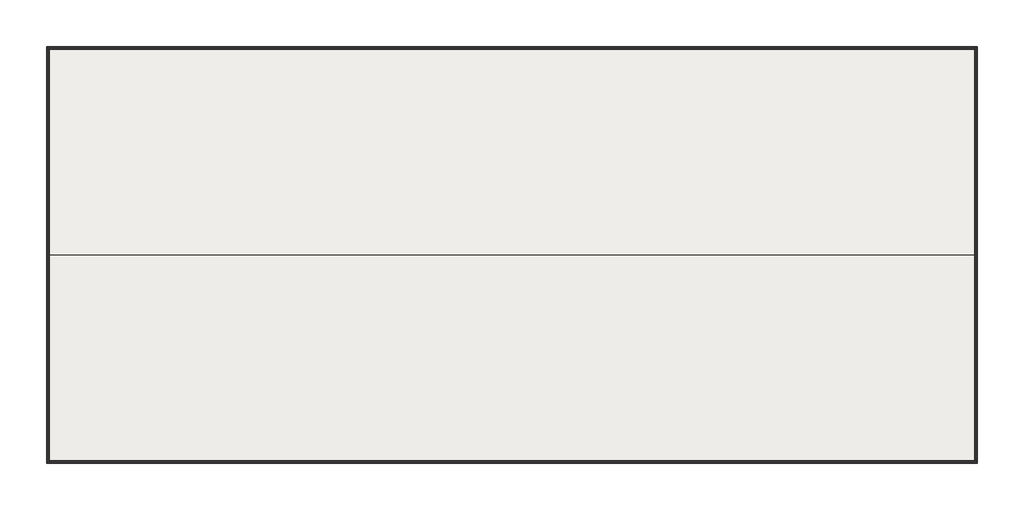
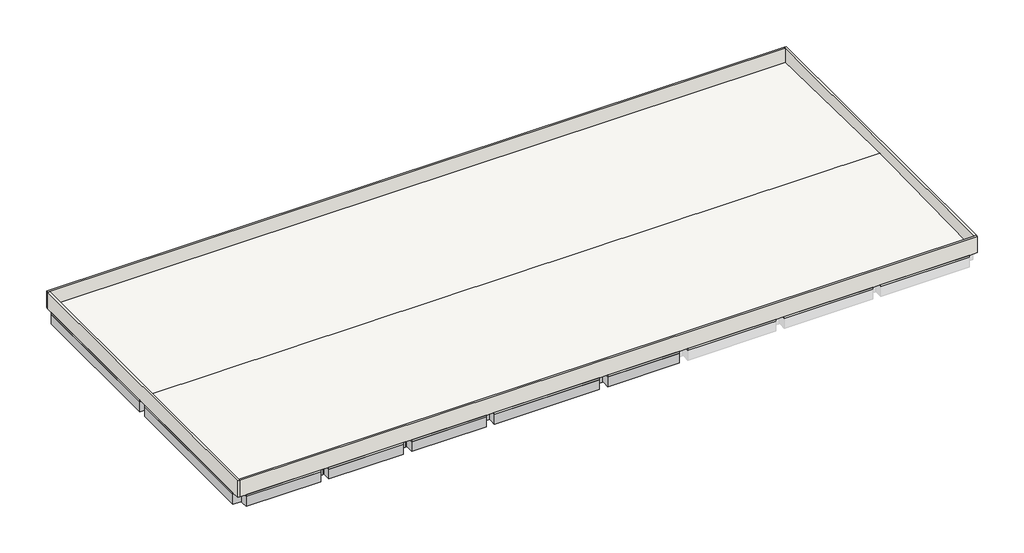
# One storey, part 1 of 2: 21 beams, 4 walls, 1 roof, 1 slab.
"""IFC4 building model written with IfcOpenShell, lengths in millimetres."""

from ifc_helpers import new_model, si_unit, frame, origin, place, context, project, spatial, polyline, outline, extrude, faceted_brep, element, save

model = new_model("IFC4")

# Units and contexts
model_context = context("Model", 3, world=origin())
ifc_project = project(units=[si_unit("LENGTHUNIT", "METRE", prefix="MILLI")], contexts=[model_context])

# Site, building, storey
site = spatial("IfcSite", under=ifc_project)
building = spatial("IfcBuilding", under=site)
storey = spatial("IfcBuildingStorey", under=building, Name="TOC", Elevation=7649.9618634)

# Beams
placement = place(None, origin())
element("IfcBeam", 1, ObjectType="RC Beam_Rectangular : H_SB_AR_S16_B600xH900_RG4", at=placement, inside=storey, context=model_context, shape_type="Brep", body=[
    faceted_brep([(300.0, 12499.5208589, 6749.9618634), (300.0, 12099.5208589, 6749.9618634), (300.0, 11899.5208589, 6749.9618634), (300.0, 11899.5208589, 7499.9618634), (300.0, 12499.5208589, 7499.9618634), (5700.0, 11899.5208589, 6749.9618634), (5700.0, 12099.5208589, 6749.9618634), (5700.0, 12499.5208589, 6749.9618634), (5700.0, 12499.5208589, 7499.9618634), (5700.0, 11899.5208589, 7499.9618634), (426.0, 11899.5208589, 7499.9618634), (2800.0, 11899.5208589, 7499.9618634), (3200.0, 11899.5208589, 7499.9618634), (3200.0, 12499.5208589, 7499.9618634), (2800.0, 12499.5208589, 7499.9618634), (426.0, 12499.5208589, 7499.9618634), (2800.0, 11899.5208589, 6749.9618634), (3200.0, 11899.5208589, 6749.9618634), (426.0, 12499.5208589, 6749.9618634), (2800.0, 12499.5208589, 6749.9618634), (3200.0, 12499.5208589, 6749.9618634)], [[[0, 1, 2, 3, 4]], [[5, 6, 7, 8, 9]], [[4, 3, 10, 11, 12, 9, 8, 13, 14, 15]], [[2, 16, 17, 5, 9, 12, 11, 10, 3]], [[2, 1, 0, 18, 19, 20, 7, 6, 5, 17, 16]], [[7, 20, 19, 18, 0, 4, 15, 14, 13, 8]]]),
])
element("IfcBeam", 2, ObjectType="RC Beam_Rectangular : H_SB_AR_S16_B600xH900_RG4", at=placement, inside=storey, context=model_context, shape_type="Brep", body=[
    faceted_brep([(6300.0, 12499.5208589, 6749.9618634), (6300.0, 12099.5208589, 6749.9618634), (6300.0, 11899.5208589, 6749.9618634), (6300.0, 11899.5208589, 7499.9618634), (6300.0, 12499.5208589, 7499.9618634), (11700.0, 11899.5208589, 6749.9618634), (11700.0, 12099.5208589, 6749.9618634), (11700.0, 12499.5208589, 6749.9618634), (11700.0, 12499.5208589, 7499.9618634), (11700.0, 11899.5208589, 7499.9618634), (8800.0, 11899.5208589, 7499.9618634), (9200.0, 11899.5208589, 7499.9618634), (9200.0, 12499.5208589, 7499.9618634), (8800.0, 12499.5208589, 7499.9618634), (8800.0, 11899.5208589, 6749.9618634), (9200.0, 11899.5208589, 6749.9618634), (8800.0, 12499.5208589, 6749.9618634), (9200.0, 12499.5208589, 6749.9618634)], [[[0, 1, 2, 3, 4]], [[5, 6, 7, 8, 9]], [[4, 3, 10, 11, 9, 8, 12, 13]], [[2, 14, 15, 5, 9, 11, 10, 3]], [[2, 1, 0, 16, 17, 7, 6, 5, 15, 14]], [[7, 17, 16, 0, 4, 13, 12, 8]]]),
])
element("IfcBeam", 3, ObjectType="RC Beam_Rectangular : H_SB_AR_S16_B600xH900_RG4", at=placement, inside=storey, context=model_context, shape_type="Brep", body=[
    faceted_brep([(12300.0, 12499.5208589, 6749.9618634), (12300.0, 12099.5208589, 6749.9618634), (12300.0, 11899.5208589, 6749.9618634), (12300.0, 11899.5208589, 7499.9618634), (12300.0, 12499.5208589, 7499.9618634), (17700.0, 11899.5208589, 6749.9618634), (17700.0, 12099.5208589, 6749.9618634), (17700.0, 12499.5208589, 6749.9618634), (17700.0, 12499.5208589, 7499.9618634), (17700.0, 11899.5208589, 7499.9618634), (14800.0, 11899.5208589, 7499.9618634), (15200.0, 11899.5208589, 7499.9618634), (15200.0, 12499.5208589, 7499.9618634), (14800.0, 12499.5208589, 7499.9618634), (14800.0, 11899.5208589, 6749.9618634), (15200.0, 11899.5208589, 6749.9618634), (14800.0, 12499.5208589, 6749.9618634), (15200.0, 12499.5208589, 6749.9618634)], [[[0, 1, 2, 3, 4]], [[5, 6, 7, 8, 9]], [[4, 3, 10, 11, 9, 8, 12, 13]], [[2, 14, 15, 5, 9, 11, 10, 3]], [[2, 1, 0, 16, 17, 7, 6, 5, 15, 14]], [[7, 17, 16, 0, 4, 13, 12, 8]]]),
])
element("IfcBeam", 4, ObjectType="RC Beam_Rectangular : H_SB_AR_S16_B600xH900_RG5", at=placement, inside=storey, context=model_context, shape_type="Brep", body=[
    faceted_brep([(26500.0, 8599.5208589, 6749.9618634), (26500.0, 8399.5208589, 6749.9618634), (26500.0, 7999.5208589, 6749.9618634), (26500.0, 7999.5208589, 7499.9618634), (26500.0, 8599.5208589, 7499.9618634), (31700.0, 7999.5208589, 6749.9618634), (31700.0, 8399.5208589, 6749.9618634), (31700.0, 8599.5208589, 6749.9618634), (31700.0, 8599.5208589, 7499.9618634), (31700.0, 7999.5208589, 7499.9618634), (28500.0, 7999.5208589, 7499.9618634), (28700.0, 7999.5208589, 7499.9618634), (28800.0, 7999.5208589, 7499.9618634), (29400.0, 7999.5208589, 7499.9618634), (29400.0, 8599.5208589, 7499.9618634), (28800.0, 8599.5208589, 7499.9618634), (28500.0, 7999.5208589, 6749.9618634), (28700.0, 7999.5208589, 6749.9618634), (28800.0, 7999.5208589, 6749.9618634), (29400.0, 7999.5208589, 6749.9618634), (28800.0, 8599.5208589, 6749.9618634), (29400.0, 8599.5208589, 6749.9618634)], [[[0, 1, 2, 3, 4]], [[5, 6, 7, 8, 9]], [[4, 3, 10, 11, 12, 13, 9, 8, 14, 15]], [[2, 16, 17, 18, 19, 5, 9, 13, 12, 11, 10, 3]], [[2, 1, 0, 20, 21, 7, 6, 5, 19, 18, 17, 16]], [[7, 21, 20, 0, 4, 15, 14, 8]]]),
])
element("IfcBeam", 5, ObjectType="RC Beam_Rectangular : H_SB_AR_S16_B600xH900_RG9", at=placement, inside=storey, context=model_context, shape_type="Brep", body=[
    faceted_brep([(300.0, 799.5208589, 6749.9618634), (300.0, 649.5208589, 6749.9618634), (300.0, 199.5208589, 6749.9618634), (300.0, 199.5208589, 7499.9618634), (300.0, 799.5208589, 7499.9618634), (5700.0, 199.5208589, 6749.9618634), (5700.0, 649.5208589, 6749.9618634), (5700.0, 799.5208589, 6749.9618634), (5700.0, 799.5208589, 7499.9618634), (5700.0, 199.5208589, 7499.9618634), (3200.0, 799.5208589, 7499.9618634), (2800.0, 799.5208589, 7499.9618634), (426.0, 799.5208589, 7499.9618634), (2800.0, 799.5208589, 6749.9618634), (3200.0, 799.5208589, 6749.9618634)], [[[0, 1, 2, 3, 4]], [[5, 6, 7, 8, 9]], [[4, 3, 9, 8, 10, 11, 12]], [[2, 5, 9, 3]], [[2, 1, 0, 13, 14, 7, 6, 5]], [[7, 14, 13, 0, 4, 12, 11, 10, 8]]]),
])
element("IfcBeam", 6, ObjectType="RC Beam_Rectangular : H_SB_AR_S16_B600xH900_RG9", at=placement, inside=storey, context=model_context, shape_type="Brep", body=[
    faceted_brep([(6300.0, 799.5208589, 6749.9618634), (6300.0, 649.5208589, 6749.9618634), (6300.0, 199.5208589, 6749.9618634), (6300.0, 199.5208589, 7499.9618634), (6300.0, 799.5208589, 7499.9618634), (11700.0, 199.5208589, 6749.9618634), (11700.0, 649.5208589, 6749.9618634), (11700.0, 799.5208589, 6749.9618634), (11700.0, 799.5208589, 7499.9618634), (11700.0, 199.5208589, 7499.9618634), (9200.0, 799.5208589, 7499.9618634), (8800.0, 799.5208589, 7499.9618634), (8800.0, 799.5208589, 6749.9618634), (9200.0, 799.5208589, 6749.9618634)], [[[0, 1, 2, 3, 4]], [[5, 6, 7, 8, 9]], [[4, 3, 9, 8, 10, 11]], [[2, 5, 9, 3]], [[2, 1, 0, 12, 13, 7, 6, 5]], [[7, 13, 12, 0, 4, 11, 10, 8]]]),
])
element("IfcBeam", 7, ObjectType="RC Beam_Rectangular : H_SB_AR_S16_B600xH900_RG9", at=placement, inside=storey, context=model_context, shape_type="Brep", body=[
    faceted_brep([(12300.0, 799.5208589, 6749.9618634), (12300.0, 649.5208589, 6749.9618634), (12300.0, 199.5208589, 6749.9618634), (12300.0, 199.5208589, 7499.9618634), (12300.0, 799.5208589, 7499.9618634), (17700.0, 199.5208589, 6749.9618634), (17700.0, 649.5208589, 6749.9618634), (17700.0, 799.5208589, 6749.9618634), (17700.0, 799.5208589, 7499.9618634), (17700.0, 199.5208589, 7499.9618634), (15200.0, 799.5208589, 7499.9618634), (14800.0, 799.5208589, 7499.9618634), (14800.0, 799.5208589, 6749.9618634), (15200.0, 799.5208589, 6749.9618634)], [[[0, 1, 2, 3, 4]], [[5, 6, 7, 8, 9]], [[4, 3, 9, 8, 10, 11]], [[2, 5, 9, 3]], [[2, 1, 0, 12, 13, 7, 6, 5]], [[7, 13, 12, 0, 4, 11, 10, 8]]]),
])
element("IfcBeam", 8, ObjectType="RC Beam_Rectangular : H_SB_AR_S16_B600xH900_RG9", at=placement, inside=storey, context=model_context, shape_type="Brep", body=[
    faceted_brep([(18300.0, 799.5208589, 6749.9618634), (18300.0, 649.5208589, 6749.9618634), (18300.0, 199.5208589, 6749.9618634), (18300.0, 199.5208589, 7499.9618634), (18300.0, 799.5208589, 7499.9618634), (25900.0, 199.5208589, 6749.9618634), (25900.0, 649.5208589, 6749.9618634), (25900.0, 799.5208589, 6749.9618634), (25900.0, 799.5208589, 7499.9618634), (25900.0, 199.5208589, 7499.9618634), (22400.0, 799.5208589, 7499.9618634), (21800.0, 799.5208589, 7499.9618634), (21800.0, 799.5208589, 6749.9618634), (22400.0, 799.5208589, 6749.9618634)], [[[0, 1, 2, 3, 4]], [[5, 6, 7, 8, 9]], [[4, 3, 9, 8, 10, 11]], [[2, 5, 9, 3]], [[2, 1, 0, 12, 13, 7, 6, 5]], [[7, 13, 12, 0, 4, 11, 10, 8]]]),
])
element("IfcBeam", 9, ObjectType="RC Beam_Rectangular : H_SB_AR_S16_B600xH900_RG9", at=placement, inside=storey, context=model_context, shape_type="Brep", body=[
    faceted_brep([(26500.0, 799.5208589, 6749.9618634), (26500.0, 649.5208589, 6749.9618634), (26500.0, 199.5208589, 6749.9618634), (26500.0, 199.5208589, 7499.9618634), (26500.0, 799.5208589, 7499.9618634), (31700.0, 199.5208589, 6749.9618634), (31700.0, 649.5208589, 6749.9618634), (31700.0, 799.5208589, 6749.9618634), (31700.0, 799.5208589, 7499.9618634), (31700.0, 199.5208589, 7499.9618634), (29400.0, 799.5208589, 7499.9618634), (28800.0, 799.5208589, 7499.9618634), (28700.0, 799.5208589, 7499.9618634), (28500.0, 799.5208589, 7499.9618634), (28800.0, 799.5208589, 6749.9618634), (29400.0, 799.5208589, 6749.9618634)], [[[0, 1, 2, 3, 4]], [[5, 6, 7, 8, 9]], [[4, 3, 9, 8, 10, 11, 12, 13]], [[2, 5, 9, 3]], [[2, 1, 0, 14, 15, 7, 6, 5]], [[7, 15, 14, 0, 4, 13, 12, 11, 10, 8]]]),
])
element("IfcBeam", 10, ObjectType="RC Beam_Rectangular : H_SB_AR_S16_B600xH900_RG6", at=placement, inside=storey, context=model_context, shape_type="Brep", body=[
    faceted_brep([(300.0, 11899.5208589, 6749.9618634), (150.0, 11899.5208589, 6749.9618634), (-300.0, 11899.5208589, 6749.9618634), (-300.0, 11899.5208589, 7499.9618634), (300.0, 11899.5208589, 7499.9618634), (-300.0, 799.5208589, 6749.9618634), (150.0, 799.5208589, 6749.9618634), (300.0, 799.5208589, 6749.9618634), (300.0, 799.5208589, 7499.9618634), (-300.0, 799.5208589, 7499.9618634)], [[[0, 1, 2, 3, 4]], [[5, 6, 7, 8, 9]], [[4, 3, 9, 8]], [[7, 0, 4, 8]], [[2, 1, 0, 7, 6, 5]], [[2, 5, 9, 3]]]),
])
element("IfcBeam", 11, ObjectType="RC Beam_Rectangular : H_SB_AR_S16_B600xH900_RG6", at=placement, inside=storey, context=model_context, shape_type="Brep", body=[
    faceted_brep([(-300.0, 12499.5208589, 6749.9618634), (150.0, 12499.5208589, 6749.9618634), (300.0, 12499.5208589, 6749.9618634), (300.0, 12499.5208589, 7499.9618634), (-300.0, 12499.5208589, 7499.9618634), (300.0, 23599.5208589, 6749.9618634), (150.0, 23599.5208589, 6749.9618634), (-300.0, 23599.5208589, 6749.9618634), (-300.0, 23599.5208589, 7499.9618634), (300.0, 23599.5208589, 7499.9618634), (300.0, 23473.5208589, 7499.9618634)], [[[0, 1, 2, 3, 4]], [[5, 6, 7, 8, 9]], [[4, 3, 10, 9, 8]], [[2, 5, 9, 10, 3]], [[2, 1, 0, 7, 6, 5]], [[7, 0, 4, 8]]]),
])
element("IfcBeam", 12, ObjectType="RC Beam_Rectangular : H_SB_AR_S16_B400xH900_RG1", at=placement, inside=storey, context=model_context, shape_type="Brep", body=[
    faceted_brep([(5800.0, 799.5208589, 7499.9618634), (6200.0, 799.5208589, 7499.9618634), (6200.0, 925.5208589, 7499.9618634), (6200.0, 11899.5208589, 7499.9618634), (5800.0, 11899.5208589, 7499.9618634), (5800.0, 925.5208589, 7499.9618634), (5800.0, 799.5208589, 6749.9618634), (6200.0, 799.5208589, 6749.9618634), (6200.0, 11899.5208589, 6749.9618634), (5800.0, 11899.5208589, 6749.9618634), (6200.0, 925.5208589, 6749.9618634), (5800.0, 925.5208589, 6749.9618634)], [[[0, 1, 2, 3, 4, 5]], [[6, 7, 1, 0]], [[8, 9, 4, 3]], [[7, 10, 8, 3, 2, 1]], [[6, 11, 9, 8, 10, 7]], [[9, 11, 6, 0, 5, 4]]]),
])
element("IfcBeam", 13, ObjectType="RC Beam_Rectangular : H_SB_AR_S16_B400xH900_RG1", at=placement, inside=storey, context=model_context, shape_type="Brep", body=[
    faceted_brep([(11800.0, 799.5208589, 7499.9618634), (12200.0, 799.5208589, 7499.9618634), (12200.0, 925.5208589, 7499.9618634), (12200.0, 11899.5208589, 7499.9618634), (11800.0, 11899.5208589, 7499.9618634), (11800.0, 925.5208589, 7499.9618634), (11800.0, 799.5208589, 6749.9618634), (12200.0, 799.5208589, 6749.9618634), (12200.0, 11899.5208589, 6749.9618634), (11800.0, 11899.5208589, 6749.9618634), (12200.0, 925.5208589, 6749.9618634), (11800.0, 925.5208589, 6749.9618634)], [[[0, 1, 2, 3, 4, 5]], [[6, 7, 1, 0]], [[8, 9, 4, 3]], [[7, 10, 8, 3, 2, 1]], [[6, 11, 9, 8, 10, 7]], [[9, 11, 6, 0, 5, 4]]]),
])
element("IfcBeam", 14, ObjectType="RC Beam_Rectangular : H_SB_AR_S16_B600xH900_RG1A", at=placement, inside=storey, context=model_context, shape_type="Brep", body=[
    faceted_brep([(17700.0, 799.5208589, 7499.9618634), (18300.0, 799.5208589, 7499.9618634), (18300.0, 925.5208589, 7499.9618634), (18300.0, 7999.5208589, 7499.9618634), (18300.0, 8599.5208589, 7499.9618634), (18300.0, 11899.5208589, 7499.9618634), (17700.0, 11899.5208589, 7499.9618634), (17700.0, 925.5208589, 7499.9618634), (17700.0, 799.5208589, 6749.9618634), (18100.0, 799.5208589, 6749.9618634), (18300.0, 799.5208589, 6749.9618634), (18300.0, 11899.5208589, 6749.9618634), (18100.0, 11899.5208589, 6749.9618634), (17700.0, 11899.5208589, 6749.9618634), (18300.0, 7999.5208589, 6749.9618634), (18300.0, 8599.5208589, 6749.9618634), (17700.0, 925.5208589, 6749.9618634)], [[[0, 1, 2, 3, 4, 5, 6, 7]], [[8, 9, 10, 1, 0]], [[11, 12, 13, 6, 5]], [[10, 14, 15, 11, 5, 4, 3, 2, 1]], [[8, 16, 13, 12, 11, 15, 14, 10, 9]], [[13, 16, 8, 0, 7, 6]]]),
])
element("IfcBeam", 15, ObjectType="RC Beam_Rectangular : H_SB_AR_S16_B500xH900_RG3", at=placement, inside=storey, context=model_context, shape_type="Brep", body=[
    faceted_brep([(26450.0, 7999.5208589, 6749.9618634), (26300.0, 7999.5208589, 6749.9618634), (26100.0, 7999.5208589, 6749.9618634), (25950.0, 7999.5208589, 6749.9618634), (25950.0, 7999.5208589, 7499.9618634), (26450.0, 7999.5208589, 7499.9618634), (25950.0, 925.5208589, 7499.9618634), (25950.0, 799.5208589, 7499.9618634), (26450.0, 799.5208589, 7499.9618634), (26450.0, 925.5208589, 7499.9618634), (26450.0, 2637.0208589, 7499.9618634), (26450.0, 2837.0208589, 7499.9618634), (25950.0, 799.5208589, 6749.9618634), (26100.0, 799.5208589, 6749.9618634), (26300.0, 799.5208589, 6749.9618634), (26450.0, 799.5208589, 6749.9618634), (26450.0, 925.5208589, 6749.9618634), (26450.0, 2637.0208589, 6749.9618634), (26450.0, 2837.0208589, 6749.9618634), (25950.0, 925.5208589, 6749.9618634)], [[[0, 1, 2, 3, 4, 5]], [[5, 4, 6, 7, 8, 9, 10, 11]], [[12, 13, 14, 15, 8, 7]], [[15, 16, 17, 18, 0, 5, 11, 10, 9, 8]], [[12, 19, 3, 2, 1, 0, 18, 17, 16, 15, 14, 13]], [[3, 19, 12, 7, 6, 4]]]),
])
element("IfcBeam", 16, ObjectType="RC Beam_Rectangular : H_SB_AR_S16_B600xH900_RG5A", at=placement, inside=storey, context=model_context, shape_type="Brep", body=[
    faceted_brep([(18300.0, 7999.5208589, 6749.9618634), (21800.0, 7999.5208589, 6749.9618634), (22400.0, 7999.5208589, 6749.9618634), (25900.0, 7999.5208589, 6749.9618634), (25900.0, 7999.5208589, 7499.9618634), (22400.0, 7999.5208589, 7499.9618634), (21800.0, 7999.5208589, 7499.9618634), (18300.0, 7999.5208589, 7499.9618634), (25900.0, 8599.5208589, 6749.9618634), (25900.0, 8399.5208589, 6749.9618634), (18300.0, 8399.5208589, 6749.9618634), (18300.0, 8599.5208589, 6749.9618634), (21800.0, 8599.5208589, 6749.9618634), (22400.0, 8599.5208589, 6749.9618634), (18300.0, 8599.5208589, 7499.9618634), (21800.0, 8599.5208589, 7499.9618634), (22400.0, 8599.5208589, 7499.9618634), (25900.0, 8599.5208589, 7499.9618634)], [[[0, 1, 2, 3, 4, 5, 6, 7]], [[8, 9, 3, 2, 1, 0, 10, 11, 12, 13]], [[8, 13, 12, 11, 14, 15, 16, 17]], [[3, 9, 8, 17, 4]], [[7, 6, 5, 4, 17, 16, 15, 14]], [[11, 10, 0, 7, 14]]]),
])
element("IfcBeam", 17, ObjectType="RC Beam_Rectangular : H_SB_AR_S16_B400xH900_RB1", at=placement, inside=storey, context=model_context, shape_type="Brep", body=[
    faceted_brep([(2800.0, 11899.5208589, 6749.9618634), (2800.0, 925.5208589, 6749.9618634), (2800.0, 799.5208589, 6749.9618634), (2800.0, 799.5208589, 7499.9618634), (2800.0, 925.5208589, 7499.9618634), (2800.0, 11899.5208589, 7499.9618634), (3200.0, 11899.5208589, 6749.9618634), (3200.0, 925.5208589, 6749.9618634), (3200.0, 799.5208589, 6749.9618634), (3200.0, 11899.5208589, 7499.9618634), (3200.0, 925.5208589, 7499.9618634), (3200.0, 799.5208589, 7499.9618634)], [[[0, 1, 2, 3, 4, 5]], [[0, 6, 7, 8, 2, 1]], [[8, 7, 6, 9, 10, 11]], [[6, 0, 5, 9]], [[2, 8, 11, 3]], [[5, 4, 3, 11, 10, 9]]]),
])
element("IfcBeam", 18, ObjectType="RC Beam_Rectangular : H_SB_AR_S16_B400xH900_RB1", at=placement, inside=storey, context=model_context, shape_type="Brep", body=[
    faceted_brep([(8800.0, 11899.5208589, 6749.9618634), (8800.0, 925.5208589, 6749.9618634), (8800.0, 799.5208589, 6749.9618634), (8800.0, 799.5208589, 7499.9618634), (8800.0, 925.5208589, 7499.9618634), (8800.0, 11899.5208589, 7499.9618634), (9200.0, 11899.5208589, 6749.9618634), (9200.0, 925.5208589, 6749.9618634), (9200.0, 799.5208589, 6749.9618634), (9200.0, 11899.5208589, 7499.9618634), (9200.0, 925.5208589, 7499.9618634), (9200.0, 799.5208589, 7499.9618634)], [[[0, 1, 2, 3, 4, 5]], [[0, 6, 7, 8, 2, 1]], [[8, 7, 6, 9, 10, 11]], [[6, 0, 5, 9]], [[2, 8, 11, 3]], [[5, 4, 3, 11, 10, 9]]]),
])
element("IfcBeam", 19, ObjectType="RC Beam_Rectangular : H_SB_AR_S16_B400xH900_RB1", at=placement, inside=storey, context=model_context, shape_type="Brep", body=[
    faceted_brep([(14800.0, 11899.5208589, 6749.9618634), (14800.0, 925.5208589, 6749.9618634), (14800.0, 799.5208589, 6749.9618634), (14800.0, 799.5208589, 7499.9618634), (14800.0, 925.5208589, 7499.9618634), (14800.0, 11899.5208589, 7499.9618634), (15200.0, 11899.5208589, 6749.9618634), (15200.0, 925.5208589, 6749.9618634), (15200.0, 799.5208589, 6749.9618634), (15200.0, 11899.5208589, 7499.9618634), (15200.0, 925.5208589, 7499.9618634), (15200.0, 799.5208589, 7499.9618634)], [[[0, 1, 2, 3, 4, 5]], [[0, 6, 7, 8, 2, 1]], [[8, 7, 6, 9, 10, 11]], [[6, 0, 5, 9]], [[2, 8, 11, 3]], [[5, 4, 3, 11, 10, 9]]]),
])
element("IfcBeam", 20, ObjectType="RC Beam_Rectangular : H_SB_AR_S16_B600xH900_RB3", at=placement, inside=storey, context=model_context, shape_type="Brep", body=[
    faceted_brep([(21800.0, 7999.5208589, 6749.9618634), (21800.0, 925.5208589, 6749.9618634), (21800.0, 799.5208589, 6749.9618634), (21800.0, 799.5208589, 7499.9618634), (21800.0, 925.5208589, 7499.9618634), (21800.0, 7999.5208589, 7499.9618634), (22400.0, 7999.5208589, 6749.9618634), (22400.0, 925.5208589, 6749.9618634), (22400.0, 799.5208589, 6749.9618634), (22400.0, 7999.5208589, 7499.9618634), (22400.0, 925.5208589, 7499.9618634), (22400.0, 799.5208589, 7499.9618634)], [[[0, 1, 2, 3, 4, 5]], [[0, 6, 7, 8, 2, 1]], [[8, 7, 6, 9, 10, 11]], [[6, 0, 5, 9]], [[2, 8, 11, 3]], [[5, 4, 3, 11, 10, 9]]]),
])
element("IfcBeam", 21, ObjectType="RC Beam_Rectangular : H_SB_AR_S16_B600xH900_RB3", at=placement, inside=storey, context=model_context, shape_type="Brep", body=[
    faceted_brep([(28800.0, 7999.5208589, 6749.9618634), (28800.0, 4999.0208589, 6749.9618634), (28800.0, 4799.0208589, 6749.9618634), (28800.0, 925.5208589, 6749.9618634), (28800.0, 799.5208589, 6749.9618634), (28800.0, 799.5208589, 7499.9618634), (28800.0, 925.5208589, 7499.9618634), (28800.0, 4799.0208589, 7499.9618634), (28800.0, 4999.0208589, 7499.9618634), (28800.0, 7999.5208589, 7499.9618634), (29400.0, 7999.5208589, 6749.9618634), (29400.0, 4999.0208589, 6749.9618634), (29400.0, 4799.0208589, 6749.9618634), (29400.0, 925.5208589, 6749.9618634), (29400.0, 799.5208589, 6749.9618634), (29400.0, 7999.5208589, 7499.9618634), (29400.0, 4999.0208589, 7499.9618634), (29400.0, 4799.0208589, 7499.9618634), (29400.0, 925.5208589, 7499.9618634), (29400.0, 799.5208589, 7499.9618634)], [[[0, 1, 2, 3, 4, 5, 6, 7, 8, 9]], [[0, 10, 11, 12, 13, 14, 4, 3, 2, 1]], [[14, 13, 12, 11, 10, 15, 16, 17, 18, 19]], [[10, 0, 9, 15]], [[4, 14, 19, 5]], [[9, 8, 7, 6, 5, 19, 18, 17, 16, 15]]]),
])

# Roof
element("IfcRoof", 22, ObjectType="H_RF_AR_B06_Mortar(Slope)_XPS_Memb_T50+120", at=placement, inside=storey, context=model_context, shape_type="SweptSolid", body=[
    extrude(outline(polyline([(24049.5208589, 7821.4618634), (24049.5208589, 7649.9618634), (349.5208589, 7649.9618634), (349.5208589, 7821.4618634), (12199.5208589, 8054.4618634), (24049.5208589, 7821.4618634)])), frame((-150.0, 0.0, 0.0), z_axis=(1.0, 0.0, 0.0), x_axis=(0.0, 1.0, 0.0)), (0.0, 0.0, 1.0), 53300.0),
])

# Slab
element("IfcSlab", 23, ObjectType="H_FL_AR_S17_Roof RC Slab_T150", at=placement, inside=storey, context=model_context, shape_type="Brep", body=[
    faceted_brep([(300.0, 11899.5208589, 7499.9618634), (300.0, 12499.5208589, 7499.9618634), (-300.0, 12499.5208589, 7499.9618634), (-300.0, 23599.5208589, 7499.9618634), (300.0, 23599.5208589, 7499.9618634), (300.0, 24199.5208589, 7499.9618634), (5700.0, 24199.5208589, 7499.9618634), (5700.0, 23599.5208589, 7499.9618634), (5800.0, 23599.5208589, 7499.9618634), (6200.0, 23599.5208589, 7499.9618634), (6300.0, 23599.5208589, 7499.9618634), (6300.0, 24199.5208589, 7499.9618634), (11700.0, 24199.5208589, 7499.9618634), (11700.0, 23599.5208589, 7499.9618634), (11800.0, 23599.5208589, 7499.9618634), (12200.0, 23599.5208589, 7499.9618634), (12300.0, 23599.5208589, 7499.9618634), (12300.0, 24199.5208589, 7499.9618634), (17700.0, 24199.5208589, 7499.9618634), (17700.0, 23599.5208589, 7499.9618634), (18300.0, 23599.5208589, 7499.9618634), (18300.0, 24199.5208589, 7499.9618634), (25900.0, 24199.5208589, 7499.9618634), (25900.0, 23599.5208589, 7499.9618634), (25950.0, 23599.5208589, 7499.9618634), (26450.0, 23599.5208589, 7499.9618634), (26500.0, 23599.5208589, 7499.9618634), (26500.0, 24199.5208589, 7499.9618634), (31700.0, 24199.5208589, 7499.9618634), (31700.0, 23599.5208589, 7499.9618634), (31750.0, 23599.5208589, 7499.9618634), (32250.0, 23599.5208589, 7499.9618634), (32300.0, 23599.5208589, 7499.9618634), (32300.0, 24199.5208589, 7499.9618634), (38700.0, 24199.5208589, 7499.9618634), (38700.0, 23599.5208589, 7499.9618634), (38750.0, 23599.5208589, 7499.9618634), (39250.0, 23599.5208589, 7499.9618634), (39300.0, 23599.5208589, 7499.9618634), (39300.0, 24199.5208589, 7499.9618634), (45700.0, 24199.5208589, 7499.9618634), (45700.0, 23599.5208589, 7499.9618634), (45750.0, 23599.5208589, 7499.9618634), (46250.0, 23599.5208589, 7499.9618634), (46300.0, 23599.5208589, 7499.9618634), (46300.0, 24199.5208589, 7499.9618634), (52700.0, 24199.5208589, 7499.9618634), (52700.0, 23599.5208589, 7499.9618634), (53300.0, 23599.5208589, 7499.9618634), (53300.0, 8599.5208589, 7499.9618634), (52700.0, 8599.5208589, 7499.9618634), (52700.0, 7999.5208589, 7499.9618634), (53300.0, 7999.5208589, 7499.9618634), (53300.0, 799.5208589, 7499.9618634), (52700.0, 799.5208589, 7499.9618634), (52700.0, 199.5208589, 7499.9618634), (46300.0, 199.5208589, 7499.9618634), (46300.0, 799.5208589, 7499.9618634), (46250.0, 799.5208589, 7499.9618634), (45750.0, 799.5208589, 7499.9618634), (45700.0, 799.5208589, 7499.9618634), (45700.0, 199.5208589, 7499.9618634), (39300.0, 199.5208589, 7499.9618634), (39300.0, 799.5208589, 7499.9618634), (39250.0, 799.5208589, 7499.9618634), (38750.0, 799.5208589, 7499.9618634), (38700.0, 799.5208589, 7499.9618634), (38700.0, 199.5208589, 7499.9618634), (32300.0, 199.5208589, 7499.9618634), (32300.0, 799.5208589, 7499.9618634), (32250.0, 799.5208589, 7499.9618634), (31750.0, 799.5208589, 7499.9618634), (31700.0, 799.5208589, 7499.9618634), (31700.0, 199.5208589, 7499.9618634), (26500.0, 199.5208589, 7499.9618634), (26500.0, 799.5208589, 7499.9618634), (26450.0, 799.5208589, 7499.9618634), (25950.0, 799.5208589, 7499.9618634), (25900.0, 799.5208589, 7499.9618634), (25900.0, 199.5208589, 7499.9618634), (18300.0, 199.5208589, 7499.9618634), (18300.0, 799.5208589, 7499.9618634), (17700.0, 799.5208589, 7499.9618634), (17700.0, 199.5208589, 7499.9618634), (12300.0, 199.5208589, 7499.9618634), (12300.0, 799.5208589, 7499.9618634), (12200.0, 799.5208589, 7499.9618634), (11800.0, 799.5208589, 7499.9618634), (11700.0, 799.5208589, 7499.9618634), (11700.0, 199.5208589, 7499.9618634), (6300.0, 199.5208589, 7499.9618634), (6300.0, 799.5208589, 7499.9618634), (6200.0, 799.5208589, 7499.9618634), (5800.0, 799.5208589, 7499.9618634), (5700.0, 799.5208589, 7499.9618634), (5700.0, 199.5208589, 7499.9618634), (300.0, 199.5208589, 7499.9618634), (300.0, 799.5208589, 7499.9618634), (-300.0, 799.5208589, 7499.9618634), (-300.0, 11899.5208589, 7499.9618634), (18300.0, 11899.5208589, 7499.9618634), (18300.0, 12499.5208589, 7499.9618634), (17700.0, 12499.5208589, 7499.9618634), (17700.0, 11899.5208589, 7499.9618634), (6300.0, 11899.5208589, 7499.9618634), (6300.0, 12499.5208589, 7499.9618634), (6200.0, 12499.5208589, 7499.9618634), (5800.0, 12499.5208589, 7499.9618634), (5700.0, 12499.5208589, 7499.9618634), (5700.0, 11899.5208589, 7499.9618634), (5800.0, 11899.5208589, 7499.9618634), (6200.0, 11899.5208589, 7499.9618634), (12300.0, 11899.5208589, 7499.9618634), (12300.0, 12499.5208589, 7499.9618634), (12200.0, 12499.5208589, 7499.9618634), (11800.0, 12499.5208589, 7499.9618634), (11700.0, 12499.5208589, 7499.9618634), (11700.0, 11899.5208589, 7499.9618634), (11800.0, 11899.5208589, 7499.9618634), (12200.0, 11899.5208589, 7499.9618634), (26500.0, 7999.5208589, 7499.9618634), (26500.0, 8599.5208589, 7499.9618634), (26450.0, 8599.5208589, 7499.9618634), (25950.0, 8599.5208589, 7499.9618634), (25900.0, 8599.5208589, 7499.9618634), (25900.0, 7999.5208589, 7499.9618634), (25950.0, 7999.5208589, 7499.9618634), (26450.0, 7999.5208589, 7499.9618634), (32300.0, 7999.5208589, 7499.9618634), (32300.0, 8599.5208589, 7499.9618634), (32250.0, 8599.5208589, 7499.9618634), (31750.0, 8599.5208589, 7499.9618634), (31700.0, 8599.5208589, 7499.9618634), (31700.0, 7999.5208589, 7499.9618634), (31750.0, 7999.5208589, 7499.9618634), (32250.0, 7999.5208589, 7499.9618634), (39300.0, 7999.5208589, 7499.9618634), (39300.0, 8599.5208589, 7499.9618634), (39250.0, 8599.5208589, 7499.9618634), (38750.0, 8599.5208589, 7499.9618634), (38700.0, 8599.5208589, 7499.9618634), (38700.0, 7999.5208589, 7499.9618634), (38750.0, 7999.5208589, 7499.9618634), (39250.0, 7999.5208589, 7499.9618634), (46300.0, 7999.5208589, 7499.9618634), (46300.0, 8599.5208589, 7499.9618634), (46250.0, 8599.5208589, 7499.9618634), (45750.0, 8599.5208589, 7499.9618634), (45700.0, 8599.5208589, 7499.9618634), (45700.0, 7999.5208589, 7499.9618634), (45750.0, 7999.5208589, 7499.9618634), (46250.0, 7999.5208589, 7499.9618634), (300.0, 12499.5208589, 7649.9618634), (300.0, 11899.5208589, 7649.9618634), (-300.0, 11899.5208589, 7649.9618634), (-300.0, 799.5208589, 7649.9618634), (300.0, 799.5208589, 7649.9618634), (300.0, 199.5208589, 7649.9618634), (5700.0, 199.5208589, 7649.9618634), (5700.0, 799.5208589, 7649.9618634), (6300.0, 799.5208589, 7649.9618634), (6300.0, 199.5208589, 7649.9618634), (11700.0, 199.5208589, 7649.9618634), (11700.0, 799.5208589, 7649.9618634), (12300.0, 799.5208589, 7649.9618634), (12300.0, 199.5208589, 7649.9618634), (17700.0, 199.5208589, 7649.9618634), (17700.0, 799.5208589, 7649.9618634), (18300.0, 799.5208589, 7649.9618634), (18300.0, 199.5208589, 7649.9618634), (25900.0, 199.5208589, 7649.9618634), (25900.0, 799.5208589, 7649.9618634), (26500.0, 799.5208589, 7649.9618634), (26500.0, 199.5208589, 7649.9618634), (31700.0, 199.5208589, 7649.9618634), (31700.0, 799.5208589, 7649.9618634), (32300.0, 799.5208589, 7649.9618634), (32300.0, 199.5208589, 7649.9618634), (38700.0, 199.5208589, 7649.9618634), (38700.0, 799.5208589, 7649.9618634), (39300.0, 799.5208589, 7649.9618634), (39300.0, 199.5208589, 7649.9618634), (45700.0, 199.5208589, 7649.9618634), (45700.0, 799.5208589, 7649.9618634), (46300.0, 799.5208589, 7649.9618634), (46300.0, 199.5208589, 7649.9618634), (52700.0, 199.5208589, 7649.9618634), (52700.0, 799.5208589, 7649.9618634), (53300.0, 799.5208589, 7649.9618634), (53300.0, 7999.5208589, 7649.9618634), (52700.0, 7999.5208589, 7649.9618634), (52700.0, 8599.5208589, 7649.9618634), (53300.0, 8599.5208589, 7649.9618634), (53300.0, 23599.5208589, 7649.9618634), (52700.0, 23599.5208589, 7649.9618634), (52700.0, 24199.5208589, 7649.9618634), (46300.0, 24199.5208589, 7649.9618634), (46300.0, 23599.5208589, 7649.9618634), (45700.0, 23599.5208589, 7649.9618634), (45700.0, 24199.5208589, 7649.9618634), (39300.0, 24199.5208589, 7649.9618634), (39300.0, 23599.5208589, 7649.9618634), (38700.0, 23599.5208589, 7649.9618634), (38700.0, 24199.5208589, 7649.9618634), (32300.0, 24199.5208589, 7649.9618634), (32300.0, 23599.5208589, 7649.9618634), (31700.0, 23599.5208589, 7649.9618634), (31700.0, 24199.5208589, 7649.9618634), (26500.0, 24199.5208589, 7649.9618634), (26500.0, 23599.5208589, 7649.9618634), (25900.0, 23599.5208589, 7649.9618634), (25900.0, 24199.5208589, 7649.9618634), (18300.0, 24199.5208589, 7649.9618634), (18300.0, 23599.5208589, 7649.9618634), (17700.0, 23599.5208589, 7649.9618634), (17700.0, 24199.5208589, 7649.9618634), (12300.0, 24199.5208589, 7649.9618634), (12300.0, 23599.5208589, 7649.9618634), (11700.0, 23599.5208589, 7649.9618634), (11700.0, 24199.5208589, 7649.9618634), (6300.0, 24199.5208589, 7649.9618634), (6300.0, 23599.5208589, 7649.9618634), (5700.0, 23599.5208589, 7649.9618634), (5700.0, 24199.5208589, 7649.9618634), (300.0, 24199.5208589, 7649.9618634), (300.0, 23599.5208589, 7649.9618634), (-300.0, 23599.5208589, 7649.9618634), (-300.0, 12499.5208589, 7649.9618634), (6300.0, 12499.5208589, 7649.9618634), (6300.0, 11899.5208589, 7649.9618634), (5700.0, 11899.5208589, 7649.9618634), (5700.0, 12499.5208589, 7649.9618634), (12300.0, 12499.5208589, 7649.9618634), (12300.0, 11899.5208589, 7649.9618634), (11700.0, 11899.5208589, 7649.9618634), (11700.0, 12499.5208589, 7649.9618634), (18300.0, 12499.5208589, 7649.9618634), (18300.0, 11899.5208589, 7649.9618634), (17700.0, 11899.5208589, 7649.9618634), (17700.0, 12499.5208589, 7649.9618634), (26500.0, 8599.5208589, 7649.9618634), (26500.0, 7999.5208589, 7649.9618634), (25900.0, 7999.5208589, 7649.9618634), (25900.0, 8599.5208589, 7649.9618634), (32300.0, 8599.5208589, 7649.9618634), (32300.0, 7999.5208589, 7649.9618634), (31700.0, 7999.5208589, 7649.9618634), (31700.0, 8599.5208589, 7649.9618634), (39300.0, 8599.5208589, 7649.9618634), (39300.0, 7999.5208589, 7649.9618634), (38700.0, 7999.5208589, 7649.9618634), (38700.0, 8599.5208589, 7649.9618634), (46300.0, 8599.5208589, 7649.9618634), (46300.0, 7999.5208589, 7649.9618634), (45700.0, 7999.5208589, 7649.9618634), (45700.0, 8599.5208589, 7649.9618634)], [[[0, 1, 2, 3, 4, 5, 6, 7, 8, 9, 10, 11, 12, 13, 14, 15, 16, 17, 18, 19, 20, 21, 22, 23, 24, 25, 26, 27, 28, 29, 30, 31, 32, 33, 34, 35, 36, 37, 38, 39, 40, 41, 42, 43, 44, 45, 46, 47, 48, 49, 50, 51, 52, 53, 54, 55, 56, 57, 58, 59, 60, 61, 62, 63, 64, 65, 66, 67, 68, 69, 70, 71, 72, 73, 74, 75, 76, 77, 78, 79, 80, 81, 82, 83, 84, 85, 86, 87, 88, 89, 90, 91, 92, 93, 94, 95, 96, 97, 98, 99], [100, 101, 102, 103], [104, 105, 106, 107, 108, 109, 110, 111], [112, 113, 114, 115, 116, 117, 118, 119], [120, 121, 122, 123, 124, 125, 126, 127], [128, 129, 130, 131, 132, 133, 134, 135], [136, 137, 138, 139, 140, 141, 142, 143], [144, 145, 146, 147, 148, 149, 150, 151]], [[152, 153, 154, 155, 156, 157, 158, 159, 160, 161, 162, 163, 164, 165, 166, 167, 168, 169, 170, 171, 172, 173, 174, 175, 176, 177, 178, 179, 180, 181, 182, 183, 184, 185, 186, 187, 188, 189, 190, 191, 192, 193, 194, 195, 196, 197, 198, 199, 200, 201, 202, 203, 204, 205, 206, 207, 208, 209, 210, 211, 212, 213, 214, 215, 216, 217, 218, 219, 220, 221, 222, 223, 224, 225, 226, 227], [228, 229, 230, 231], [232, 233, 234, 235], [236, 237, 238, 239], [240, 241, 242, 243], [244, 245, 246, 247], [248, 249, 250, 251], [252, 253, 254, 255]], [[48, 193, 192, 49]], [[52, 189, 188, 53]], [[157, 96, 95, 158]], [[161, 90, 89, 162]], [[165, 84, 83, 166]], [[169, 80, 79, 170]], [[173, 74, 73, 174]], [[177, 68, 67, 178]], [[181, 62, 61, 182]], [[185, 56, 55, 186]], [[154, 99, 98, 155]], [[2, 227, 226, 3]], [[5, 224, 223, 6]], [[11, 220, 219, 12]], [[17, 216, 215, 18]], [[21, 212, 211, 22]], [[27, 208, 207, 28]], [[33, 204, 203, 34]], [[39, 200, 199, 40]], [[45, 196, 195, 46]], [[0, 153, 152, 1]], [[153, 0, 99, 154]], [[1, 152, 227, 2]], [[104, 229, 228, 105]], [[229, 104, 111, 110, 109, 230]], [[230, 109, 108, 231]], [[231, 108, 107, 106, 105, 228]], [[112, 233, 232, 113]], [[233, 112, 119, 118, 117, 234]], [[234, 117, 116, 235]], [[235, 116, 115, 114, 113, 232]], [[100, 237, 236, 101]], [[237, 100, 103, 238]], [[238, 103, 102, 239]], [[239, 102, 101, 236]], [[4, 225, 224, 5]], [[225, 4, 3, 226]], [[10, 221, 220, 11]], [[221, 10, 9, 8, 7, 222]], [[222, 7, 6, 223]], [[16, 217, 216, 17]], [[217, 16, 15, 14, 13, 218]], [[218, 13, 12, 219]], [[20, 213, 212, 21]], [[213, 20, 19, 214]], [[214, 19, 18, 215]], [[26, 209, 208, 27]], [[209, 26, 25, 24, 23, 210]], [[210, 23, 22, 211]], [[32, 205, 204, 33]], [[205, 32, 31, 30, 29, 206]], [[206, 29, 28, 207]], [[38, 201, 200, 39]], [[201, 38, 37, 36, 35, 202]], [[202, 35, 34, 203]], [[44, 197, 196, 45]], [[197, 44, 43, 42, 41, 198]], [[198, 41, 40, 199]], [[47, 194, 193, 48]], [[194, 47, 46, 195]], [[120, 241, 240, 121]], [[241, 120, 127, 126, 125, 242]], [[242, 125, 124, 243]], [[243, 124, 123, 122, 121, 240]], [[128, 245, 244, 129]], [[245, 128, 135, 134, 133, 246]], [[246, 133, 132, 247]], [[247, 132, 131, 130, 129, 244]], [[136, 249, 248, 137]], [[249, 136, 143, 142, 141, 250]], [[250, 141, 140, 251]], [[251, 140, 139, 138, 137, 248]], [[144, 253, 252, 145]], [[253, 144, 151, 150, 149, 254]], [[254, 149, 148, 255]], [[255, 148, 147, 146, 145, 252]], [[51, 190, 189, 52]], [[190, 51, 50, 191]], [[191, 50, 49, 192]], [[156, 97, 96, 157]], [[97, 156, 155, 98]], [[160, 91, 90, 161]], [[94, 159, 158, 95]], [[159, 94, 93, 92, 91, 160]], [[164, 85, 84, 165]], [[88, 163, 162, 89]], [[163, 88, 87, 86, 85, 164]], [[168, 81, 80, 169]], [[82, 167, 166, 83]], [[167, 82, 81, 168]], [[172, 75, 74, 173]], [[78, 171, 170, 79]], [[171, 78, 77, 76, 75, 172]], [[176, 69, 68, 177]], [[72, 175, 174, 73]], [[175, 72, 71, 70, 69, 176]], [[180, 63, 62, 181]], [[66, 179, 178, 67]], [[179, 66, 65, 64, 63, 180]], [[184, 57, 56, 185]], [[60, 183, 182, 61]], [[183, 60, 59, 58, 57, 184]], [[54, 187, 186, 55]], [[187, 54, 53, 188]]]),
])

# Walls
element("IfcWall", 24, ObjectType="H_WA_AR_B02_Ext Wall_RC T150", at=placement, inside=storey, context=model_context, shape_type="Brep", body=[
    faceted_brep([(-300.0, 24049.5208589, 7649.9618634), (-150.0, 24049.5208589, 7649.9618634), (53150.0, 24049.5208589, 7649.9618634), (53150.0, 24049.5208589, 7821.4618634), (53150.0, 24049.5208589, 8899.9618634), (-150.0, 24049.5208589, 8899.9618634), (-300.0, 24049.5208589, 8899.9618634), (-300.0, 24199.5208589, 7649.9618634), (-300.0, 24199.5208589, 8899.9618634), (53150.0, 24199.5208589, 8899.9618634), (53150.0, 24199.5208589, 7649.9618634), (52700.0, 24199.5208589, 7649.9618634), (46300.0, 24199.5208589, 7649.9618634), (45700.0, 24199.5208589, 7649.9618634), (39300.0, 24199.5208589, 7649.9618634), (38700.0, 24199.5208589, 7649.9618634), (32300.0, 24199.5208589, 7649.9618634), (31700.0, 24199.5208589, 7649.9618634), (26500.0, 24199.5208589, 7649.9618634), (25900.0, 24199.5208589, 7649.9618634), (18300.0, 24199.5208589, 7649.9618634), (17700.0, 24199.5208589, 7649.9618634), (12300.0, 24199.5208589, 7649.9618634), (11700.0, 24199.5208589, 7649.9618634), (6300.0, 24199.5208589, 7649.9618634), (5700.0, 24199.5208589, 7649.9618634), (300.0, 24199.5208589, 7649.9618634)], [[[0, 1, 2, 3, 4, 5, 6]], [[7, 8, 9, 10, 11, 12, 13, 14, 15, 16, 17, 18, 19, 20, 21, 22, 23, 24, 25, 26]], [[2, 1, 0, 7, 26, 25, 24, 23, 22, 21, 20, 19, 18, 17, 16, 15, 14, 13, 12, 11, 10]], [[6, 5, 4, 9, 8]], [[0, 6, 8, 7]], [[4, 3, 2, 10, 9]]]),
])
element("IfcWall", 25, ObjectType="H_WA_AR_B02_Ext Wall_RC T150", at=placement, inside=storey, context=model_context, shape_type="Brep", body=[
    faceted_brep([(-150.0, 199.5208589, 7649.9618634), (-150.0, 349.5208589, 7649.9618634), (-150.0, 24049.5208589, 7649.9618634), (-150.0, 24049.5208589, 7821.4618634), (-150.0, 24049.5208589, 8899.9618634), (-150.0, 349.5208589, 8899.9618634), (-150.0, 199.5208589, 8899.9618634), (-300.0, 199.5208589, 7649.9618634), (-300.0, 199.5208589, 8899.9618634), (-300.0, 24049.5208589, 8899.9618634), (-300.0, 24049.5208589, 7649.9618634), (-300.0, 23599.5208589, 7649.9618634), (-300.0, 12499.5208589, 7649.9618634), (-300.0, 11899.5208589, 7649.9618634), (-300.0, 799.5208589, 7649.9618634)], [[[0, 1, 2, 3, 4, 5, 6]], [[7, 8, 9, 10, 11, 12, 13, 14]], [[2, 1, 0, 7, 14, 13, 12, 11, 10]], [[6, 5, 4, 9, 8]], [[0, 6, 8, 7]], [[4, 3, 2, 10, 9]]]),
])
element("IfcWall", 26, ObjectType="H_WA_AR_B02_Ext Wall_RC T150", at=placement, inside=storey, context=model_context, shape_type="Brep", body=[
    faceted_brep([(53300.0, 349.5208589, 7649.9618634), (53150.0, 349.5208589, 7649.9618634), (-150.0, 349.5208589, 7649.9618634), (-150.0, 349.5208589, 7821.4618634), (-150.0, 349.5208589, 8899.9618634), (53150.0, 349.5208589, 8899.9618634), (53300.0, 349.5208589, 8899.9618634), (53300.0, 199.5208589, 7649.9618634), (53300.0, 199.5208589, 8899.9618634), (-150.0, 199.5208589, 8899.9618634), (-150.0, 199.5208589, 7649.9618634), (300.0, 199.5208589, 7649.9618634), (5700.0, 199.5208589, 7649.9618634), (6300.0, 199.5208589, 7649.9618634), (11700.0, 199.5208589, 7649.9618634), (12300.0, 199.5208589, 7649.9618634), (17700.0, 199.5208589, 7649.9618634), (18300.0, 199.5208589, 7649.9618634), (25900.0, 199.5208589, 7649.9618634), (26500.0, 199.5208589, 7649.9618634), (31700.0, 199.5208589, 7649.9618634), (32300.0, 199.5208589, 7649.9618634), (38700.0, 199.5208589, 7649.9618634), (39300.0, 199.5208589, 7649.9618634), (45700.0, 199.5208589, 7649.9618634), (46300.0, 199.5208589, 7649.9618634), (52700.0, 199.5208589, 7649.9618634)], [[[0, 1, 2, 3, 4, 5, 6]], [[7, 8, 9, 10, 11, 12, 13, 14, 15, 16, 17, 18, 19, 20, 21, 22, 23, 24, 25, 26]], [[2, 1, 0, 7, 26, 25, 24, 23, 22, 21, 20, 19, 18, 17, 16, 15, 14, 13, 12, 11, 10]], [[6, 5, 4, 9, 8]], [[0, 6, 8, 7]], [[4, 3, 2, 10, 9]]]),
])
element("IfcWall", 27, ObjectType="H_WA_AR_B02_Ext Wall_RC T150", at=placement, inside=storey, context=model_context, shape_type="Brep", body=[
    faceted_brep([(53150.0, 24199.5208589, 7649.9618634), (53150.0, 24049.5208589, 7649.9618634), (53150.0, 349.5208589, 7649.9618634), (53150.0, 349.5208589, 7821.4618634), (53150.0, 349.5208589, 8899.9618634), (53150.0, 24049.5208589, 8899.9618634), (53150.0, 24199.5208589, 8899.9618634), (53300.0, 24199.5208589, 7649.9618634), (53300.0, 24199.5208589, 8899.9618634), (53300.0, 349.5208589, 8899.9618634), (53300.0, 349.5208589, 7649.9618634), (53300.0, 799.5208589, 7649.9618634), (53300.0, 7999.5208589, 7649.9618634), (53300.0, 8599.5208589, 7649.9618634), (53300.0, 23599.5208589, 7649.9618634)], [[[0, 1, 2, 3, 4, 5, 6]], [[7, 8, 9, 10, 11, 12, 13, 14]], [[2, 1, 0, 7, 14, 13, 12, 11, 10]], [[6, 5, 4, 9, 8]], [[0, 6, 8, 7]], [[4, 3, 2, 10, 9]]]),
])

save(model, "model.ifc")

# Revit data of these elements
# Type "RC Beam_Rectangular : H_SB_AR_S16_B600xH900_RG4"
#   중앙부 하부근 = ""
#   중앙부 상부근 = ""
#   중앙부 보조근 = ""
#   중앙부 늑근 = ""
#   외단부 하부근 = ""
#   외단부 상부근 = ""
#   외단부 보조근 = ""
#   외단부 늑근 = ""
#   부호 = "TG3"
#   내단부 하부근 = ""
#   내단부 상부근 = ""
#   내단부 보조근 = ""
#   내단부 늑근 = ""
#   ALL 하부근 = "3-D20"
#   ALL 상부근 = "3-D20"
#   ALL 보조근 = ""
#   ALL 늑근 = "2-D10 @120"
#   Width = 600 mm
#   Height = 900 mm
#   Length [instance default] = 1524 mm
#   b = 600 mm
#   h = 900 mm
#   hec_material3 [instance default] = none
#   hec_material2 [instance default] = none
#   hec_material1 [instance default] = none
#   Structural Material [instance default] = none
#   Assembly Code = ""
# Type "RC Beam_Rectangular : H_SB_AR_S16_B600xH900_RG5"
#   중앙부 하부근 = ""
#   중앙부 상부근 = ""
#   중앙부 보조근 = ""
#   중앙부 늑근 = ""
#   외단부 하부근 = ""
#   외단부 상부근 = ""
#   외단부 보조근 = ""
#   외단부 늑근 = ""
#   부호 = "TG3"
#   내단부 하부근 = ""
#   내단부 상부근 = ""
#   내단부 보조근 = ""
#   내단부 늑근 = ""
#   ALL 하부근 = "3-D20"
#   ALL 상부근 = "3-D20"
#   ALL 보조근 = ""
#   ALL 늑근 = "2-D10 @120"
#   Width = 600 mm
#   Height = 900 mm
#   Length [instance default] = 1524 mm
#   b = 600 mm
#   h = 900 mm
#   hec_material3 [instance default] = none
#   hec_material2 [instance default] = none
#   hec_material1 [instance default] = none
#   Structural Material [instance default] = none
#   Assembly Code = ""
# Type "RC Beam_Rectangular : H_SB_AR_S16_B600xH900_RG9"
#   중앙부 하부근 = ""
#   중앙부 상부근 = ""
#   중앙부 보조근 = ""
#   중앙부 늑근 = ""
#   외단부 하부근 = ""
#   외단부 상부근 = ""
#   외단부 보조근 = ""
#   외단부 늑근 = ""
#   부호 = "TG3"
#   내단부 하부근 = ""
#   내단부 상부근 = ""
#   내단부 보조근 = ""
#   내단부 늑근 = ""
#   ALL 하부근 = "3-D20"
#   ALL 상부근 = "3-D20"
#   ALL 보조근 = ""
#   ALL 늑근 = "2-D10 @120"
#   Width = 600 mm
#   Height = 900 mm
#   Length [instance default] = 1524 mm
#   b = 600 mm
#   h = 900 mm
#   hec_material3 [instance default] = none
#   hec_material2 [instance default] = none
#   hec_material1 [instance default] = none
#   Structural Material [instance default] = none
#   Assembly Code = ""
# Type "RC Beam_Rectangular : H_SB_AR_S16_B600xH900_RG6"
#   중앙부 하부근 = ""
#   중앙부 상부근 = ""
#   중앙부 보조근 = ""
#   중앙부 늑근 = ""
#   외단부 하부근 = ""
#   외단부 상부근 = ""
#   외단부 보조근 = ""
#   외단부 늑근 = ""
#   부호 = "TG3"
#   내단부 하부근 = ""
#   내단부 상부근 = ""
#   내단부 보조근 = ""
#   내단부 늑근 = ""
#   ALL 하부근 = "3-D20"
#   ALL 상부근 = "3-D20"
#   ALL 보조근 = ""
#   ALL 늑근 = "2-D10 @120"
#   Width = 600 mm
#   Height = 900 mm
#   Length [instance default] = 1524 mm
#   b = 600 mm
#   h = 900 mm
#   hec_material3 [instance default] = none
#   hec_material2 [instance default] = none
#   hec_material1 [instance default] = none
#   Structural Material [instance default] = none
#   Assembly Code = ""
# Type "RC Beam_Rectangular : H_SB_AR_S16_B400xH900_RG1"
#   중앙부 하부근 = ""
#   중앙부 상부근 = ""
#   중앙부 보조근 = ""
#   중앙부 늑근 = ""
#   외단부 하부근 = ""
#   외단부 상부근 = ""
#   외단부 보조근 = ""
#   외단부 늑근 = ""
#   부호 = "TG3"
#   내단부 하부근 = ""
#   내단부 상부근 = ""
#   내단부 보조근 = ""
#   내단부 늑근 = ""
#   ALL 하부근 = "3-D20"
#   ALL 상부근 = "3-D20"
#   ALL 보조근 = ""
#   ALL 늑근 = "2-D10 @120"
#   Width = 400 mm
#   Height = 900 mm
#   Length [instance default] = 1524 mm
#   b = 400 mm
#   h = 900 mm
#   hec_material3 [instance default] = none
#   hec_material2 [instance default] = none
#   hec_material1 [instance default] = none
#   Structural Material [instance default] = none
#   Assembly Code = ""
# Type "RC Beam_Rectangular : H_SB_AR_S16_B600xH900_RG1A"
#   중앙부 하부근 = ""
#   중앙부 상부근 = ""
#   중앙부 보조근 = ""
#   중앙부 늑근 = ""
#   외단부 하부근 = ""
#   외단부 상부근 = ""
#   외단부 보조근 = ""
#   외단부 늑근 = ""
#   부호 = "TG3"
#   내단부 하부근 = ""
#   내단부 상부근 = ""
#   내단부 보조근 = ""
#   내단부 늑근 = ""
#   ALL 하부근 = "3-D20"
#   ALL 상부근 = "3-D20"
#   ALL 보조근 = ""
#   ALL 늑근 = "2-D10 @120"
#   Width = 600 mm
#   Height = 900 mm
#   Length [instance default] = 1524 mm
#   b = 600 mm
#   h = 900 mm
#   hec_material3 [instance default] = none
#   hec_material2 [instance default] = none
#   hec_material1 [instance default] = none
#   Structural Material [instance default] = none
#   Assembly Code = ""
# Type "RC Beam_Rectangular : H_SB_AR_S16_B500xH900_RG3"
#   중앙부 하부근 = ""
#   중앙부 상부근 = ""
#   중앙부 보조근 = ""
#   중앙부 늑근 = ""
#   외단부 하부근 = ""
#   외단부 상부근 = ""
#   외단부 보조근 = ""
#   외단부 늑근 = ""
#   부호 = "TG3"
#   내단부 하부근 = ""
#   내단부 상부근 = ""
#   내단부 보조근 = ""
#   내단부 늑근 = ""
#   ALL 하부근 = "3-D20"
#   ALL 상부근 = "3-D20"
#   ALL 보조근 = ""
#   ALL 늑근 = "2-D10 @120"
#   Width = 500 mm
#   Height = 900 mm
#   Length [instance default] = 1524 mm
#   b = 500 mm
#   h = 900 mm
#   hec_material3 [instance default] = none
#   hec_material2 [instance default] = none
#   hec_material1 [instance default] = none
#   Structural Material [instance default] = none
#   Assembly Code = ""
# Type "RC Beam_Rectangular : H_SB_AR_S16_B600xH900_RG5A"
#   중앙부 하부근 = ""
#   중앙부 상부근 = ""
#   중앙부 보조근 = ""
#   중앙부 늑근 = ""
#   외단부 하부근 = ""
#   외단부 상부근 = ""
#   외단부 보조근 = ""
#   외단부 늑근 = ""
#   부호 = "TG3"
#   내단부 하부근 = ""
#   내단부 상부근 = ""
#   내단부 보조근 = ""
#   내단부 늑근 = ""
#   ALL 하부근 = "3-D20"
#   ALL 상부근 = "3-D20"
#   ALL 보조근 = ""
#   ALL 늑근 = "2-D10 @120"
#   Width = 600 mm
#   Height = 900 mm
#   Length [instance default] = 1524 mm
#   b = 600 mm
#   h = 900 mm
#   hec_material3 [instance default] = none
#   hec_material2 [instance default] = none
#   hec_material1 [instance default] = none
#   Structural Material [instance default] = none
#   Assembly Code = ""
# Type "RC Beam_Rectangular : H_SB_AR_S16_B400xH900_RB1"
#   중앙부 하부근 = ""
#   중앙부 상부근 = ""
#   중앙부 보조근 = ""
#   중앙부 늑근 = ""
#   외단부 하부근 = ""
#   외단부 상부근 = ""
#   외단부 보조근 = ""
#   외단부 늑근 = ""
#   부호 = "TG3"
#   내단부 하부근 = ""
#   내단부 상부근 = ""
#   내단부 보조근 = ""
#   내단부 늑근 = ""
#   ALL 하부근 = "3-D20"
#   ALL 상부근 = "3-D20"
#   ALL 보조근 = ""
#   ALL 늑근 = "2-D10 @120"
#   Width = 400 mm
#   Height = 900 mm
#   Length [instance default] = 1524 mm
#   b = 400 mm
#   h = 900 mm
#   hec_material3 [instance default] = none
#   hec_material2 [instance default] = none
#   hec_material1 [instance default] = none
#   Structural Material [instance default] = none
#   Assembly Code = ""
# Type "RC Beam_Rectangular : H_SB_AR_S16_B600xH900_RB3"
#   중앙부 하부근 = ""
#   중앙부 상부근 = ""
#   중앙부 보조근 = ""
#   중앙부 늑근 = ""
#   외단부 하부근 = ""
#   외단부 상부근 = ""
#   외단부 보조근 = ""
#   외단부 늑근 = ""
#   부호 = "TG3"
#   내단부 하부근 = ""
#   내단부 상부근 = ""
#   내단부 보조근 = ""
#   내단부 늑근 = ""
#   ALL 하부근 = "3-D20"
#   ALL 상부근 = "3-D20"
#   ALL 보조근 = ""
#   ALL 늑근 = "2-D10 @120"
#   Width = 600 mm
#   Height = 900 mm
#   Length [instance default] = 1524 mm
#   b = 600 mm
#   h = 900 mm
#   hec_material3 [instance default] = none
#   hec_material2 [instance default] = none
#   hec_material1 [instance default] = none
#   Structural Material [instance default] = none
#   Assembly Code = ""
# Type "H_RF_AR_B06_Mortar(Slope)_XPS_Memb_T50+120"
#   Layers, outside or top first: 1.5 mm "Roofing - EPDM Membrane" (function 4); 120 mm "00_Insulation_Rigid_hec" (function 3); 50 mm "Slab, Screed" (function 1)
# Type "H_FL_AR_S17_Roof RC Slab_T150"
#   Keynote = ""
#   Type Comments = ""
#   Description = ""
#   Function = 1
#   Layers, outside or top first: 150 mm "Concrete - Cast-in-Place Concrete - 35 MPa" (function 1)
# Type "H_WA_AR_B02_Ext Wall_RC T150"
#   Type Comments = ""
#   Layers, outside or top first: 150 mm "Concrete - Cast-in-Place Concrete - 35 MPa" (function 1)
# Elements 1, 2, 3 (IfcBeam, "RC Beam_Rectangular : H_SB_AR_S16_B600xH900_RG4")
#   Comments = ""
#   hec_material3 = none
#   hec_material2 = none
#   hec_material1 = none
#   Structural Material = Concrete - Cast-in-Place Concrete - 35 MPa
#   Phase Created = New Construction
#   Materials on its faces: "Concrete - Cast-in-Place Concrete - 35 MPa"
# Element 4 (IfcBeam, "RC Beam_Rectangular : H_SB_AR_S16_B600xH900_RG5")
#   Comments = ""
#   hec_material3 = none
#   hec_material2 = none
#   hec_material1 = none
#   Structural Material = Concrete - Cast-in-Place Concrete - 35 MPa
#   Phase Created = New Construction
#   Materials on its faces: "Concrete - Cast-in-Place Concrete - 35 MPa"
# Elements 5, 6, 7, 8, 9 (IfcBeam, "RC Beam_Rectangular : H_SB_AR_S16_B600xH900_RG9")
#   Comments = ""
#   hec_material3 = none
#   hec_material2 = none
#   hec_material1 = none
#   Structural Material = Concrete - Cast-in-Place Concrete - 35 MPa
#   Phase Created = New Construction
#   Materials on its faces: "Concrete - Cast-in-Place Concrete - 35 MPa"
# Elements 10, 11 (IfcBeam, "RC Beam_Rectangular : H_SB_AR_S16_B600xH900_RG6")
#   Comments = ""
#   hec_material3 = none
#   hec_material2 = none
#   hec_material1 = none
#   Structural Material = Concrete - Cast-in-Place Concrete - 35 MPa
#   Phase Created = New Construction
#   Materials on its faces: "Concrete - Cast-in-Place Concrete - 35 MPa"
# Elements 12, 13 (IfcBeam, "RC Beam_Rectangular : H_SB_AR_S16_B400xH900_RG1")
#   Comments = ""
#   hec_material3 = none
#   hec_material2 = none
#   hec_material1 = none
#   Structural Material = Concrete - Cast-in-Place Concrete - 35 MPa
#   Phase Created = New Construction
#   Materials on its faces: "Concrete - Cast-in-Place Concrete - 35 MPa"
# Element 14 (IfcBeam, "RC Beam_Rectangular : H_SB_AR_S16_B600xH900_RG1A")
#   Comments = ""
#   hec_material3 = none
#   hec_material2 = none
#   hec_material1 = none
#   Structural Material = Concrete - Cast-in-Place Concrete - 35 MPa
#   Phase Created = New Construction
#   Materials on its faces: "Concrete - Cast-in-Place Concrete - 35 MPa"
# Element 15 (IfcBeam, "RC Beam_Rectangular : H_SB_AR_S16_B500xH900_RG3")
#   Comments = ""
#   hec_material3 = none
#   hec_material2 = none
#   hec_material1 = none
#   Structural Material = Concrete - Cast-in-Place Concrete - 35 MPa
#   Phase Created = New Construction
#   Materials on its faces: "Concrete - Cast-in-Place Concrete - 35 MPa"
# Element 16 (IfcBeam, "RC Beam_Rectangular : H_SB_AR_S16_B600xH900_RG5A")
#   hec_material3 = none
#   hec_material2 = none
#   hec_material1 = none
#   Structural Material = Concrete - Cast-in-Place Concrete - 35 MPa
#   Phase Created = New Construction
#   Materials on its faces: "Concrete - Cast-in-Place Concrete - 35 MPa"
# Elements 17, 18, 19 (IfcBeam, "RC Beam_Rectangular : H_SB_AR_S16_B400xH900_RB1")
#   hec_material3 = none
#   hec_material2 = none
#   hec_material1 = none
#   Structural Material = Concrete - Cast-in-Place Concrete - 35 MPa
#   Phase Created = New Construction
#   Materials on its faces: "Concrete - Cast-in-Place Concrete - 35 MPa"
# Elements 20, 21 (IfcBeam, "RC Beam_Rectangular : H_SB_AR_S16_B600xH900_RB3")
#   hec_material3 = none
#   hec_material2 = none
#   hec_material1 = none
#   Structural Material = Concrete - Cast-in-Place Concrete - 35 MPa
#   Phase Created = New Construction
#   Materials on its faces: "Concrete - Cast-in-Place Concrete - 35 MPa"
# Element 22 (IfcRoof, "H_RF_AR_B06_Mortar(Slope)_XPS_Memb_T50+120")
#   H_Roof Style Name = "Concrete Slab(Slope)+Insulation+Protection Concrete+Waterproofing"
#   H_Roof_Base Material = "Concrete Slab"
#   H_Roof_Finish-1 = "Liquid Waterproofing"
#   H_Roof_Finish-2 = "Rigid Extruded Polystyrene Foam Insulation(XPS)"
#   H_Roof_Finish-3 = "Welded Wire Fabric"
#   H_Roof_Finish-4 = "Protective Concrete w/ Steel Trowel Finish"
#   H_Roof_Finish-5 = "스카이패널 건식복합방수"
#   H_Roof_Style Remark = "* 스카이패널 건식복합방수 : WM 없음"
#   built-in parameter 1001705 = 25.661 (stored number, unit not read)
#   built-in parameter 1001710 = 33615
#   H_Roof Style No = RF41
#   Phase Created = New Construction
#   Materials on its faces: "Slab, Screed", "Roofing - EPDM Membrane"
# Element 23 (IfcSlab, "H_FL_AR_S17_Roof RC Slab_T150")
#   Comments = ""
#   TMP_Element Name = "SS2"
#   Height Offset From Level = 0 mm
#   built-in parameter 1001954 = 1
#   Phase Created = New Construction
#   Materials on its faces: "Concrete - Cast-in-Place Concrete - 35 MPa"
# Elements 24, 25, 26, 27 (IfcWall, "H_WA_AR_B02_Ext Wall_RC T150")
#   Top Offset = 0 mm
#   Base Offset = 0 mm
#   wall height = 1250 mm
#   Phase Created = New Construction
#   Base Constraint = TOC
#   Top Constraint = TOP
#   Materials on its faces: "Concrete - Cast-in-Place Concrete - 35 MPa"
# Materials
#   "Roofing - EPDM Membrane": class "Plastic", colour RGB 127 127 127, transparency 0, Description = "Exterior finish, roofing"
#   "00_Insulation_Rigid_hec": class "Insulation", colour RGB 255 255 217, transparency 0, Description = "Insulation(Rigid)", Cost = 0
#   "Slab, Screed": class "Concrete", colour RGB 120 120 120, transparency 0, Description = "Concrete slab topping", Cost = 0
#   "Concrete - Cast-in-Place Concrete - 35 MPa": class "Concrete", colour RGB 192 192 192, transparency 0, Cost = 0
